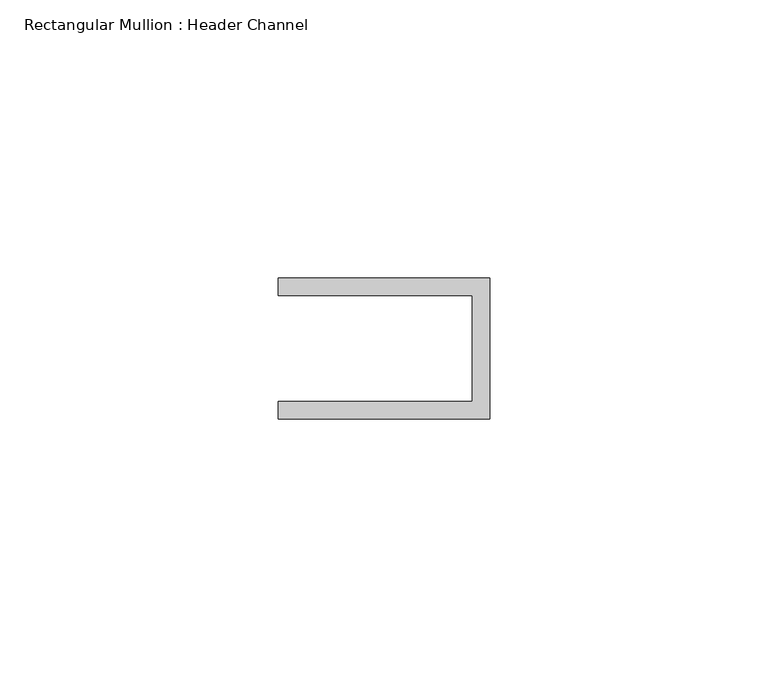
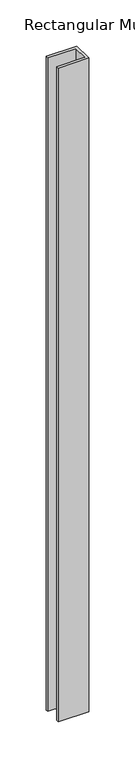
"""IFC4 building model written with IfcOpenShell, lengths in millimetres: member geometry, Rectangular Mullion : Header Channel."""

import ifcopenshell
import ifcopenshell.guid

model = None  # the IFC model being written
_history = None  # IfcOwnerHistory: only IFC2X3 demands one
_inside = {}  # id of a spatial element -> (the spatial element, [elements in it])
_under = {}  # id of a project, library or spatial element -> (it, [spatial elements below it])
_declared = {}  # id of a project -> (the project, [libraries it declares])
_typed = {}  # id of a type object -> (the type object, [elements of that type])
_made_of = {}  # id of a material, layer set ... -> (it, [elements and type objects made of it])


def new_model(schema):
    """Start an empty IFC model of exactly this schema.

    Asked for "IFC4X3", IfcOpenShell would pick the latest addendum, in which some entities
    have other attributes; the version numbers below select the first issue.
    IFC2X3 requires an IfcOwnerHistory on every rooted entity: one is made here for all.
    """
    global model, _history
    if schema == "IFC4X3":
        model = ifcopenshell.file(schema_version=(4, 3, 0, 0))
    else:
        model = ifcopenshell.file(schema=schema)
    _inside.clear()
    _under.clear()
    _declared.clear()
    _typed.clear()
    _made_of.clear()
    _history = None
    if model.schema == "IFC2X3":
        org = make("IfcOrganization", Name="unknown")
        user = make(
            "IfcPersonAndOrganization",
            ThePerson=make("IfcPerson", FamilyName="unknown"),
            TheOrganization=org,
        )
        app = make(
            "IfcApplication",
            ApplicationDeveloper=org,
            Version="unknown",
            ApplicationFullName="unknown",
            ApplicationIdentifier="unknown",
        )
        _history = make(
            "IfcOwnerHistory",
            OwningUser=user,
            OwningApplication=app,
            ChangeAction="ADDED",
            CreationDate=0,
        )
    return model


def make(cls, **values):
    """One entity of the class cls with the attributes given. An attribute that is None is left unset."""
    return model.create_entity(
        cls, **{name: value for name, value in values.items() if value is not None}
    )


def rooted(cls, **values):
    """An entity with a GlobalId (a new one), such as an element, a storey or a relation."""
    return make(cls, GlobalId=ifcopenshell.guid.new(), OwnerHistory=_history, **values)


def si_unit(unit_type, name, prefix=None):
    """IfcSIUnit, for example si_unit("LENGTHUNIT", "METRE", prefix="MILLI")."""
    return make("IfcSIUnit", UnitType=unit_type, Prefix=prefix, Name=name)


def assignment(units):
    """IfcUnitAssignment: the units of a project."""
    return None if units is None else make("IfcUnitAssignment", Units=units)


def point(xyz):
    """IfcCartesianPoint."""
    return None if xyz is None else make("IfcCartesianPoint", Coordinates=xyz)


def direction(xyz):
    """IfcDirection."""
    return None if xyz is None else make("IfcDirection", DirectionRatios=xyz)


def frame(location, z_axis=None, x_axis=None):
    """IfcAxis2Placement3D, a coordinate frame: its origin and axes. An axis left out is left unset."""
    return make(
        "IfcAxis2Placement3D",
        Location=point(location),
        Axis=direction(z_axis),
        RefDirection=direction(x_axis),
    )


def origin():
    """The frame at (0, 0, 0) with its axes left unset."""
    return frame((0.0, 0.0, 0.0))


def place(relative_to, where):
    """IfcLocalPlacement: puts the frame where relative to a parent placement (None: the world)."""
    return make(
        "IfcLocalPlacement", PlacementRelTo=relative_to, RelativePlacement=where
    )


def context(
    kind, dimensions, precision=None, world=None, true_north=None, identifier=None
):
    """IfcGeometricRepresentationContext, for example the 3D "Model" context."""
    return make(
        "IfcGeometricRepresentationContext",
        ContextIdentifier=identifier,
        ContextType=kind,
        CoordinateSpaceDimension=dimensions,
        Precision=precision,
        WorldCoordinateSystem=world,
        TrueNorth=true_north,
    )


def project(units=None, contexts=None):
    """IfcProject with its units and contexts."""
    return rooted(
        "IfcProject",
        Name="project",
        RepresentationContexts=contexts,
        UnitsInContext=assignment(units),
    )


def spatial(cls, under=None, at=None, **own):
    """A site, building, storey or space (cls), placed at a placement, below another one or the project."""
    s = rooted(cls, ObjectPlacement=at, **own)
    if under is not None:
        _under.setdefault(under.id(), (under, []))[1].append(s)
    return s


def polyline(points):
    """IfcPolyline through the points."""
    return make("IfcPolyline", Points=[point(p) for p in points])


def outline(outer, holes=None, kind="AREA"):
    """IfcArbitraryClosedProfileDef: a profile drawn as a closed curve; with holes, ...WithVoids."""
    if holes is None:
        return make("IfcArbitraryClosedProfileDef", ProfileType=kind, OuterCurve=outer)
    return make(
        "IfcArbitraryProfileDefWithVoids",
        ProfileType=kind,
        OuterCurve=outer,
        InnerCurves=holes,
    )


def extrude(swept, where, along, depth):
    """IfcExtrudedAreaSolid: the profile swept, set in the frame where, extruded along a direction by depth."""
    return make(
        "IfcExtrudedAreaSolid",
        SweptArea=swept,
        Position=where,
        ExtrudedDirection=direction(along),
        Depth=depth,
    )


def shape(context_of_items, identifier, shape_type, items):
    """IfcShapeRepresentation: the items that make up one representation, for example the "Body"."""
    return make(
        "IfcShapeRepresentation",
        ContextOfItems=context_of_items,
        RepresentationIdentifier=identifier,
        RepresentationType=shape_type,
        Items=items,
    )


def source(mapping_origin, context_of_items, identifier, shape_type, items):
    """IfcRepresentationMap: a shape defined once, which mapped items show again and again."""
    return make(
        "IfcRepresentationMap",
        MappingOrigin=mapping_origin,
        MappedRepresentation=shape(context_of_items, identifier, shape_type, items),
    )


def transform(
    local_origin,
    x_axis=None,
    y_axis=None,
    z_axis=None,
    scale=None,
    scale2=None,
    scale3=None,
    uniform=True,
):
    """IfcCartesianTransformationOperator3D, or its non-uniform kind. x_axis, y_axis, z_axis: its Axis1, 2, 3."""
    if uniform:
        return make(
            "IfcCartesianTransformationOperator3D",
            Axis1=direction(x_axis),
            Axis2=direction(y_axis),
            LocalOrigin=point(local_origin),
            Scale=scale,
            Axis3=direction(z_axis),
        )
    return make(
        "IfcCartesianTransformationOperator3DnonUniform",
        Axis1=direction(x_axis),
        Axis2=direction(y_axis),
        LocalOrigin=point(local_origin),
        Scale=scale,
        Axis3=direction(z_axis),
        Scale2=scale2,
        Scale3=scale3,
    )


def mapped(mapping_source, mapping_target):
    """IfcMappedItem: shows the shape of a source again, moved by a transform."""
    return make(
        "IfcMappedItem", MappingSource=mapping_source, MappingTarget=mapping_target
    )


def made_of(thing, what):
    """Note that an element or type object is made of a material, layer set ...; save() writes the relation."""
    if what is not None:
        _made_of.setdefault(what.id(), (what, []))[1].append(thing)
    return thing


def element(
    cls,
    number,
    at=None,
    inside=None,
    cuts=None,
    type_object=None,
    material=None,
    context=None,
    identifier="Body",
    shape_type=None,
    held_by="IfcProductDefinitionShape",
    body=None,
    shapes=None,
    **own,
):
    """One element of the class cls, such as IfcWall. Its Tag is "e" and its number.

    at: its placement. inside: the storey or other place that contains it. cuts: it is an
    opening in that element (IfcRelVoidsElement). A single representation is given by context,
    identifier, shape_type and body (its items); several are given by shapes. held_by: the class
    of the entity that holds the representations. save() writes the other relations.
    """
    e = rooted(cls, Tag="e%d" % number, ObjectPlacement=at, **own)
    if body is not None:
        shapes = [shape(context, identifier, shape_type, body)]
    if shapes is not None:
        e.Representation = make(held_by, Representations=shapes)
    if inside is not None:
        _inside.setdefault(inside.id(), (inside, []))[1].append(e)
    if cuts is not None:
        rooted(
            "IfcRelVoidsElement", RelatingBuildingElement=cuts, RelatedOpeningElement=e
        )
    if type_object is not None:
        _typed.setdefault(type_object.id(), (type_object, []))[1].append(e)
    return made_of(e, material)


def aggregate(whole, parts):
    """IfcRelAggregates: a whole, such as a stair, and the parts it consists of."""
    return rooted("IfcRelAggregates", RelatingObject=whole, RelatedObjects=parts)


def save(model, path):
    """Write the relations noted so far, then the file.

    IfcRelAggregates (storeys below a building ...), IfcRelContainedInSpatialStructure (elements
    in a storey), IfcRelDefinesByType, IfcRelAssociatesMaterial and IfcRelDeclares: one each for
    every whole, place, type object, material and project.
    """
    for whole, parts in _under.values():
        aggregate(whole, parts)
    for where, things in _inside.values():
        rooted(
            "IfcRelContainedInSpatialStructure",
            RelatedElements=things,
            RelatingStructure=where,
        )
    for kind, things in _typed.values():
        rooted("IfcRelDefinesByType", RelatedObjects=things, RelatingType=kind)
    for what, things in _made_of.values():
        rooted("IfcRelAssociatesMaterial", RelatedObjects=things, RelatingMaterial=what)
    for by, libraries in _declared.values():
        rooted("IfcRelDeclares", RelatingContext=by, RelatedDefinitions=libraries)
    model.write(path)


def rectangular_mullion_header_channel_8741caab(model_context):
    return source(origin(), model_context, "Body", "SweptSolid", [
        extrude(outline(polyline([(0.0, -12.7), (-38.1, -12.7), (-38.1, -9.525), (-3.175, -9.525), (-3.175, 9.525), (-38.1, 9.525), (-38.1, 12.7), (0.0, 12.7), (0.0, -12.7)])), frame((0.0, 0.0, -862.0125), z_axis=(0.0, 0.0, 1.0), x_axis=(1.0, 0.0, 0.0)), (0.0, 0.0, 1.0), 862.0125),
    ])


if __name__ == "__main__":
    model = new_model("IFC4")
    model_context = context("Model", 3, world=origin())
    ifc_project = project(units=[si_unit("LENGTHUNIT", "METRE", prefix="MILLI")], contexts=[model_context])
    site = spatial("IfcSite", under=ifc_project)
    building = spatial("IfcBuilding", under=site)
    placement = place(None, origin())
    rectangular_mullion_header_channel_shape = rectangular_mullion_header_channel_8741caab(model_context)
    element("IfcMember", 1, ObjectType="Rectangular Mullion : Header Channel", at=placement, inside=building, context=model_context, shape_type="MappedRepresentation", body=[
        mapped(rectangular_mullion_header_channel_shape, transform((0.0, 0.0, 0.0), x_axis=(1.0, 0.0, 0.0), y_axis=(0.0, 1.0, 0.0), z_axis=(0.0, 0.0, 1.0))),
    ])
    save(model, "model.ifc")

# Revit data of these elements
# Type "Rectangular Mullion : Header Channel"
#   built-in parameter 1007322 = 0.0833333 (stored number, unit not read)
#   built-in parameter 1007321 = -0.03125 (stored number, unit not read)
#   built-in parameter 1007320 = 0.0416667 (stored number, unit not read)
# Element 1 (IfcMember, "Rectangular Mullion : Header Channel")
#   Materials on its faces: "ALUM"
# Materials
#   "ALUM": class "Generic", colour RGB 157 157 157, transparency 0, Cost = 0
